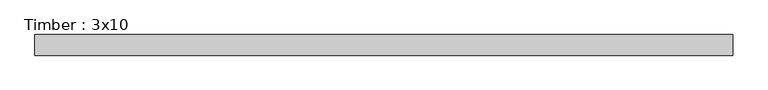
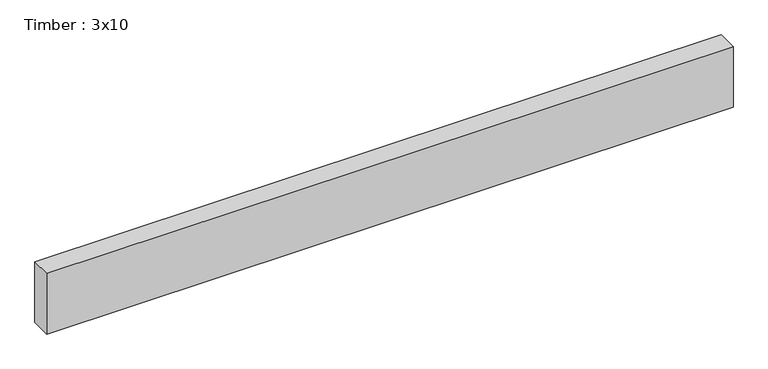
"""IFC4 building model written with IfcOpenShell, lengths in millimetres: beam geometry, Timber : 3x10."""

from ifc_helpers import new_model, si_unit, frame, origin, place, context, project, spatial, polyline, outline, extrude, source, transform, mapped, element, save


def timber_3x10_b3201cc8(model_context):
    return source(origin(), model_context, "Body", "SweptSolid", [
        extrude(outline(polyline([(1384.2999994, 38.1), (1384.2999994, -38.1), (-1197.0684633, -38.1), (-1197.0684633, 38.1), (1384.2999994, 38.1)])), frame((0.0, 0.0, -120.65), z_axis=(0.0, 0.0, 1.0), x_axis=(1.0, 0.0, 0.0)), (0.0, 0.0, 1.0), 241.3),
    ])


if __name__ == "__main__":
    model = new_model("IFC4")
    model_context = context("Model", 3, world=origin())
    ifc_project = project(units=[si_unit("LENGTHUNIT", "METRE", prefix="MILLI")], contexts=[model_context])
    site = spatial("IfcSite", under=ifc_project)
    building = spatial("IfcBuilding", under=site)
    placement = place(None, origin())
    timber_3x10_shape = timber_3x10_b3201cc8(model_context)
    element("IfcBeam", 1, ObjectType="Timber : 3x10", at=placement, inside=building, context=model_context, shape_type="MappedRepresentation", body=[
        mapped(timber_3x10_shape, transform((0.0, 0.0, 0.0), x_axis=(1.0, 0.0, 0.0), y_axis=(0.0, 1.0, 0.0), z_axis=(0.0, 0.0, 1.0))),
    ])
    save(model, "model.ifc")

# Revit data of these elements
# Type "Timber : 3x10"
#   Assembly Code = "B10"
#   A = 0.362847 SF
#   Length [instance default] = 5' - 0"
#   b = 0' - 3"
#   d = 0' - 9 1/2"
#   Structural Material [instance default] = Softwood, Lumber
# Element 1 (IfcBeam, "Timber : 3x10")
#   Materials on its faces: "Softwood, Lumber"
# Materials
#   "Softwood, Lumber": class "Wood", colour RGB 144 113 62, transparency 0, Description = "Pinus Echinata", Cost = 0
